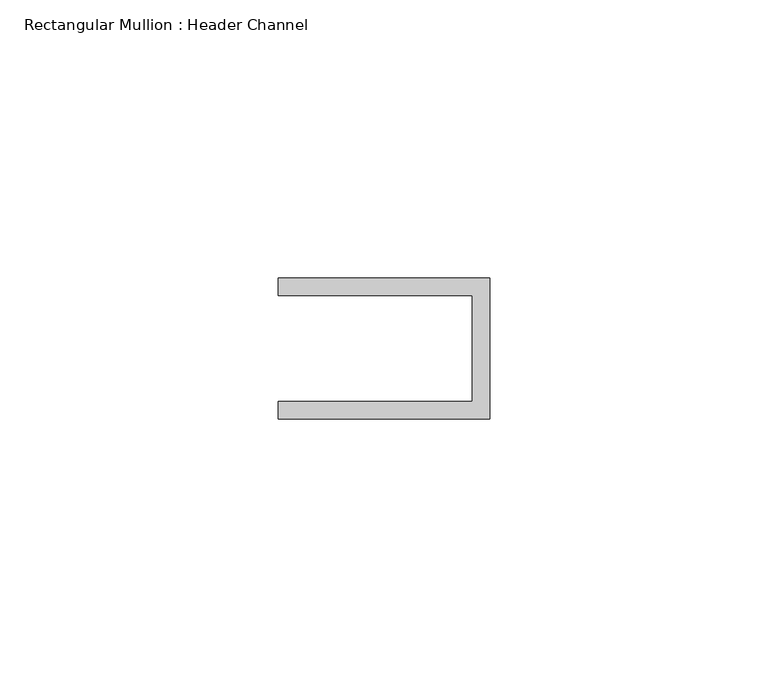
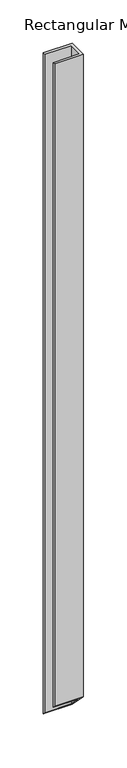
"""IFC4 building model written with IfcOpenShell, lengths in millimetres: member geometry, Rectangular Mullion : Header Channel."""

from ifc_helpers import new_model, si_unit, origin, place, context, project, spatial, faceted_brep, source, transform, mapped, element, save


def rectangular_mullion_header_channel_44dfd35a(model_context):
    return source(origin(), model_context, "Body", "Brep", [
        faceted_brep([(0.0, -12.7, 0.0), (0.0, 12.7, 0.0), (-38.1, 12.7, 0.0), (-38.1, 9.525, 0.0), (-3.175, 9.525, 0.0), (-3.175, -9.525, 0.0), (-38.1, -9.525, 0.0), (-38.1, -12.7, 0.0), (0.0, -12.7, -901.7000003), (0.0, 12.7, -927.1000003), (-38.1, 12.7, -927.1000003), (-38.1, 9.525, -923.9250003), (-3.175, 9.525, -923.9250003), (-3.175, -9.525, -904.8750003), (-38.1, -9.525, -904.8750003), (-38.1, -12.7, -901.7000003)], [[[0, 1, 2, 3, 4, 5, 6, 7]], [[1, 0, 8, 9]], [[2, 1, 9, 10]], [[3, 2, 10, 11]], [[4, 3, 11, 12]], [[5, 4, 12, 13]], [[6, 5, 13, 14]], [[7, 6, 14, 15]], [[0, 7, 15, 8]], [[8, 15, 14, 13, 12, 11, 10, 9]]]),
    ])


if __name__ == "__main__":
    model = new_model("IFC4")
    model_context = context("Model", 3, world=origin())
    ifc_project = project(units=[si_unit("LENGTHUNIT", "METRE", prefix="MILLI")], contexts=[model_context])
    site = spatial("IfcSite", under=ifc_project)
    building = spatial("IfcBuilding", under=site)
    placement = place(None, origin())
    rectangular_mullion_header_channel_shape = rectangular_mullion_header_channel_44dfd35a(model_context)
    element("IfcMember", 1, ObjectType="Rectangular Mullion : Header Channel", at=placement, inside=building, context=model_context, shape_type="MappedRepresentation", body=[
        mapped(rectangular_mullion_header_channel_shape, transform((0.0, 0.0, 0.0), x_axis=(1.0, 0.0, 0.0), y_axis=(0.0, 1.0, 0.0), z_axis=(0.0, 0.0, 1.0))),
    ])
    save(model, "model.ifc")

# Revit data of these elements
# Type "Rectangular Mullion : Header Channel"
#   built-in parameter 1007322 = 0.0833333 (stored number, unit not read)
#   built-in parameter 1007321 = -0.03125 (stored number, unit not read)
#   built-in parameter 1007320 = 0.0416667 (stored number, unit not read)
# Element 1 (IfcMember, "Rectangular Mullion : Header Channel")
#   Materials on its faces: "ALUM"
# Materials
#   "ALUM": class "Generic", colour RGB 157 157 157, transparency 0, Cost = 0
